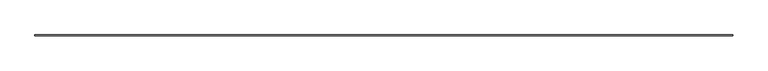
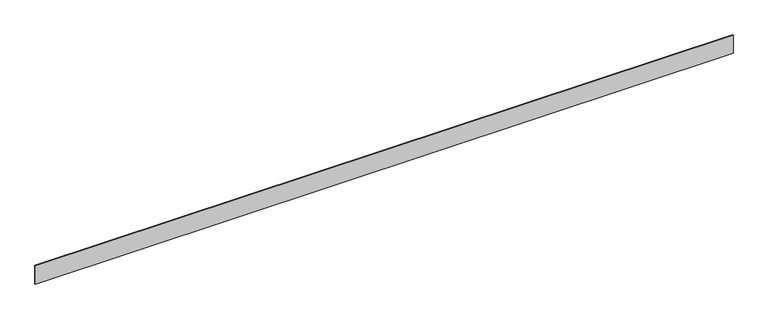
"""IFC4 building model written with IfcOpenShell, lengths in millimetres: proxy geometry, Generic Models 7:Generic Models 1:6:Generic Models 1:6 : Generic Models 7:Generic Models 1:337419:2 : Generic Models 7:Generic Models 1:6:Generic Models 1:6 : Generic Models 7:Generic Models 1:337419:312901."""

from ifc_helpers import new_model, si_unit, frame, origin, place, context, project, spatial, polyline, outline, extrude, source, transform, mapped, element, save


def generic_models_e25939af(model_context):
    return source(origin(), model_context, "Body", "SweptSolid", [
        extrude(outline(polyline([(-579089.5913841, -3.1687897), (-579089.5913841, -1222.375), (-579140.3913841, -1222.375), (-579140.3913841, -5.2854564), (-579089.5913841, -3.1687897)])), frame((557809.7867239, 0.0, 0.0), z_axis=(1.0, 0.0, 0.0), x_axis=(0.0, 1.0, 0.0)), (0.0, 0.0, 1.0), 44500.8),
    ])


if __name__ == "__main__":
    model = new_model("IFC4")
    model_context = context("Model", 3, world=origin())
    ifc_project = project(units=[si_unit("LENGTHUNIT", "METRE", prefix="MILLI")], contexts=[model_context])
    site = spatial("IfcSite", under=ifc_project)
    building = spatial("IfcBuilding", under=site)
    placement = place(None, origin())
    generic_models_shape = generic_models_e25939af(model_context)
    element("IfcBuildingElementProxy", 1, Name="Generic Models 7:Generic Models 1:6:Generic Models 1:6 : Generic Models 7:Generic Models 1:337419:2 : Generic Models 7:Generic Models 1:6:Generic Models 1:6 : Generic Models 7:Generic Models 1:337419:312901", ObjectType="Generic Models 7:Generic Models 1:6:Generic Models 1:6 : Generic Models 7:Generic Models 1:337419:2 : Generic Models 7:Generic Models 1:6:Generic Models 1:6 : Generic Models 7:Generic Models 1:337419:312901", at=placement, inside=building, context=model_context, shape_type="MappedRepresentation", body=[
        mapped(generic_models_shape, transform((0.0, 0.0, 0.0), x_axis=(1.0, 0.0, 0.0), y_axis=(0.0, 1.0, 0.0), z_axis=(0.0, 0.0, 1.0))),
    ])
    save(model, "model.ifc")

# Revit data of these elements
# Type "Generic Models 7:Generic Models 1:6:Generic Models 1:6 : Generic Models 7:Generic Models 1:337419:2 : Generic Models 7:Generic Models 1:6:Generic Models 1:6 : Generic Models 7:Generic Models 1:337419:312901"
#   NameOverride = "Generic Models 7:Generic Models 1:6:Generic Models 1:6 : Generic Models 7:Generic Models 1:337419:312901"
#   ObjectTypeOverride = "Generic Models 1:6 : Generic Models 7:Generic Models 1:337419"
#   Reference = "Generic Models 1"
#   Tag = "312901"
# Element 1 (IfcBuildingElementProxy, "Generic Models 7:Generic Models 1:6:Generic Models 1:6 : Generic Models 7:Generic Models 1:337419:2 : Generic Models 7:Generic Models 1:6:Generic Models 1:6 : Generic Models 7:Generic Models 1:337419:312901")
#   Materials on its faces: "EXTRUDED POLYSTYRENE (XPS) RIGID FOAM INSULATION (FOAMULAR® 250 OR SIMILAR)"
# Materials
#   "EXTRUDED POLYSTYRENE (XPS) RIGID FOAM INSULATION (FOAMULAR® 250 OR SIMILAR)": class "Unassigned", colour RGB 247 185 194, transparency 0, Cost = 0
